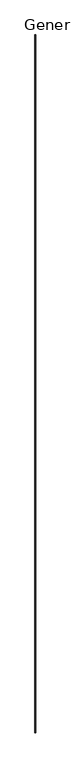
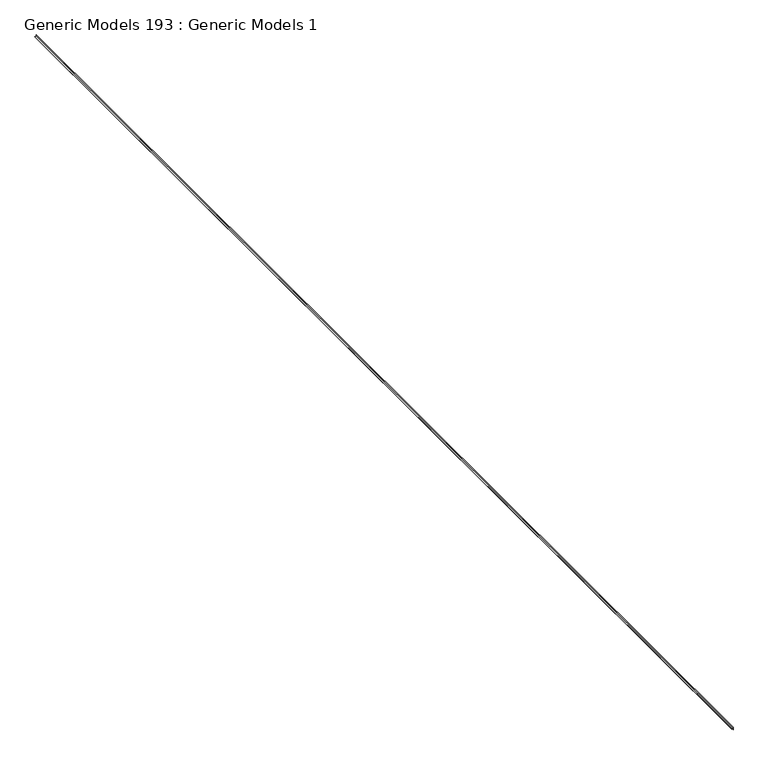
"""IFC4 building model written with IfcOpenShell, lengths in millimetres: proxy geometry, Generic Models 193 : Generic Models 1."""

from ifc_helpers import new_model, si_unit, frame, origin, place, context, project, spatial, polyline, outline, extrude, source, transform, mapped, element, save


def generic_models_193_generic_models_1_dbaa7c81(model_context):
    return source(origin(), model_context, "Body", "SweptSolid", [
        extrude(outline(polyline([(126375.541, -8999.7331401), (126375.541, -9001.0031401), (126356.491, -9001.0031401), (126356.491, -9021.9581401), (126351.7412, -9021.9581401), (126351.7412, -9020.6881401), (126355.221, -9020.6881401), (126355.221, -9001.0031401), (126336.171, -9001.0031401), (126336.171, -8999.7331401), (126375.541, -8999.7331401)])), frame((0.0, -7068.1230338, 0.0), z_axis=(0.0, 1.0, 0.0), x_axis=(0.0, 0.0, 1.0)), (0.0, 0.0, 1.0), 19050.0),
    ])


if __name__ == "__main__":
    model = new_model("IFC4")
    model_context = context("Model", 3, world=origin())
    ifc_project = project(units=[si_unit("LENGTHUNIT", "METRE", prefix="MILLI")], contexts=[model_context])
    site = spatial("IfcSite", under=ifc_project)
    building = spatial("IfcBuilding", under=site)
    placement = place(None, origin())
    generic_models_193_generic_models_1_shape = generic_models_193_generic_models_1_dbaa7c81(model_context)
    element("IfcBuildingElementProxy", 1, Name="Generic Models 193 : Generic Models 1", ObjectType="Generic Models 193 : Generic Models 1", at=placement, inside=building, context=model_context, shape_type="MappedRepresentation", body=[
        mapped(generic_models_193_generic_models_1_shape, transform((0.0, 0.0, 0.0), x_axis=(1.0, 0.0, 0.0), y_axis=(0.0, 1.0, 0.0), z_axis=(0.0, 0.0, 1.0))),
    ])
    save(model, "model.ifc")

# Revit data of these elements
# Element 1 (IfcBuildingElementProxy, "Generic Models 193 : Generic Models 1")
#   Materials on its faces: "_ 16 GA. COPPER VENTED T REVEAL BEAD (CONT. AROUND PERIMETER OF BEAM)"
# Materials
#   "_ 16 GA. COPPER VENTED T REVEAL BEAD (CONT. AROUND PERIMETER OF BEAM)": class "Generic", colour RGB 253 192 103, transparency 0, Cost = 0
